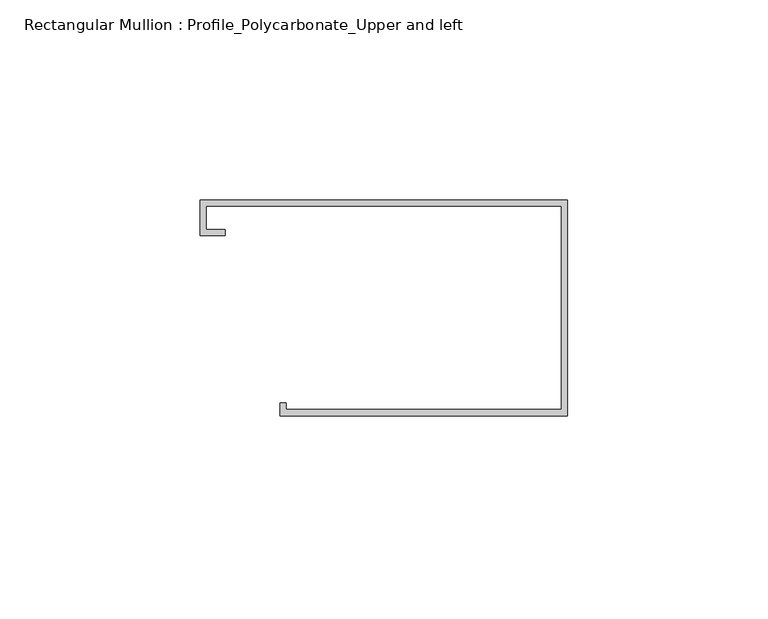
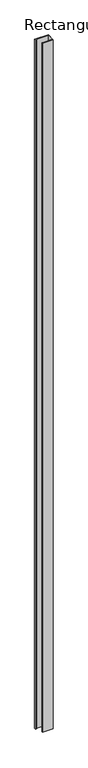
"""IFC4 building model written with IfcOpenShell, lengths in millimetres: member geometry, Rectangular Mullion : Profile_Polycarbonate_Upper and left."""

from ifc_helpers import new_model, si_unit, frame, origin, place, context, project, spatial, polyline, outline, extrude, source, transform, mapped, element, save


def rectangular_mullion_profile_polycarbonate_upper_and_left_e18db48f(model_context):
    return source(origin(), model_context, "Body", "SweptSolid", [
        extrude(outline(polyline([(0.0, 28.984575), (0.0, -25.015825), (-71.9836, -25.015825), (-71.9836, -21.840825), (-70.3961, -21.840825), (-70.3961, -23.428325), (-1.5875, -23.428325), (-1.5875, 27.397075), (-90.4113, 27.397075), (-90.4113, 21.580475), (-85.6488, 21.580475), (-85.6488, 19.992975), (-91.9988, 19.992975), (-91.9988, 28.984575), (0.0, 28.984575)])), frame((0.0, 0.0, -4876.8), z_axis=(0.0, 0.0, 1.0), x_axis=(1.0, 0.0, 0.0)), (0.0, 0.0, 1.0), 4876.8),
    ])


if __name__ == "__main__":
    model = new_model("IFC4")
    model_context = context("Model", 3, world=origin())
    ifc_project = project(units=[si_unit("LENGTHUNIT", "METRE", prefix="MILLI")], contexts=[model_context])
    site = spatial("IfcSite", under=ifc_project)
    building = spatial("IfcBuilding", under=site)
    placement = place(None, origin())
    rectangular_mullion_profile_polycarbonate_upper_and_left_shape = rectangular_mullion_profile_polycarbonate_upper_and_left_e18db48f(model_context)
    element("IfcMember", 1, ObjectType="Rectangular Mullion : Profile_Polycarbonate_Upper and left", at=placement, inside=building, context=model_context, shape_type="MappedRepresentation", body=[
        mapped(rectangular_mullion_profile_polycarbonate_upper_and_left_shape, transform((0.0, 0.0, 0.0), x_axis=(1.0, 0.0, 0.0), y_axis=(0.0, 1.0, 0.0), z_axis=(0.0, 0.0, 1.0))),
    ])
    save(model, "model.ifc")

# Revit data of these elements
# Type "Rectangular Mullion : Profile_Polycarbonate_Upper and left"
#   built-in parameter 1007322 = 0.177167 (stored number, unit not read)
#   built-in parameter 1007321 = 0.00520833 (stored number, unit not read)
#   built-in parameter 1007320 = 0 (stored number, unit not read)
